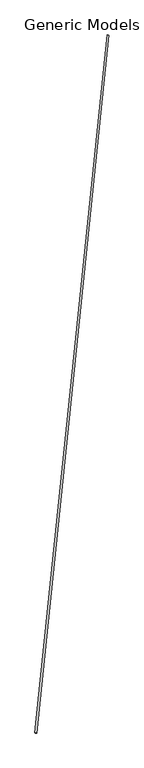
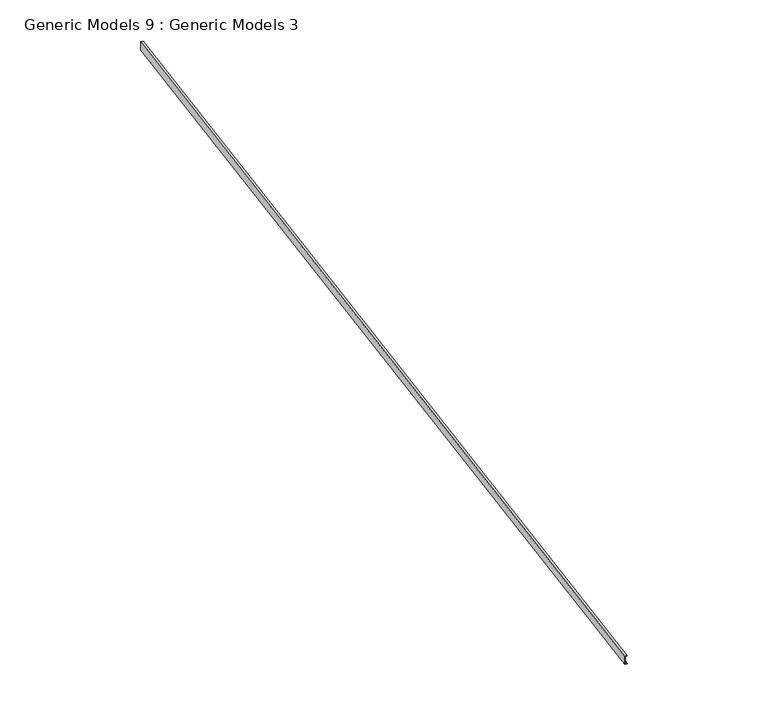
"""IFC4 building model written with IfcOpenShell, lengths in millimetres: proxy geometry, Generic Models 9 : Generic Models 3."""

from ifc_helpers import new_model, si_unit, frame, origin, place, context, project, spatial, polyline, outline, extrude, source, transform, mapped, element, save


def generic_models_9_generic_models_3_2757e302(model_context):
    return source(origin(), model_context, "Body", "SweptSolid", [
        extrude(outline(polyline([(44.6902649, 0.0), (44.6902649, -12.700212), (43.1027649, -12.7002121), (43.1027649, -1.5875), (1.5874999, -1.5875), (1.5875, -12.7), (-1e-07, -12.7), (0.0, 0.0), (44.6902649, 0.0)])), frame((34217.1785108, 30921.6063685, 271737.307868), z_axis=(-0.10293344407674772, -0.9946674410191907, 0.006433340254794664), x_axis=(0.0006724680329078983, 0.006398105948638647, 0.9999793057993824)), (0.0, 0.0, 1.0), 5311.9304914),
    ])


if __name__ == "__main__":
    model = new_model("IFC4")
    model_context = context("Model", 3, world=origin())
    ifc_project = project(units=[si_unit("LENGTHUNIT", "METRE", prefix="MILLI")], contexts=[model_context])
    site = spatial("IfcSite", under=ifc_project)
    building = spatial("IfcBuilding", under=site)
    placement = place(None, origin())
    generic_models_9_generic_models_3_shape = generic_models_9_generic_models_3_2757e302(model_context)
    element("IfcBuildingElementProxy", 1, Name="Generic Models 9 : Generic Models 3", ObjectType="Generic Models 9 : Generic Models 3", at=placement, inside=building, context=model_context, shape_type="MappedRepresentation", body=[
        mapped(generic_models_9_generic_models_3_shape, transform((0.0, 0.0, 0.0), x_axis=(1.0, 0.0, 0.0), y_axis=(0.0, 1.0, 0.0), z_axis=(0.0, 0.0, 1.0))),
    ])
    save(model, "model.ifc")

# Revit data of these elements
# Element 1 (IfcBuildingElementProxy, "Generic Models 9 : Generic Models 3")
#   Materials on its faces: "GALV. BRAKE METAL - (COLOR: MATCH ALUM. WINDOWS)"
# Materials
#   "GALV. BRAKE METAL - (COLOR: MATCH ALUM. WINDOWS)": class "Generic", colour RGB 234 234 234, transparency 0, Cost = 0
